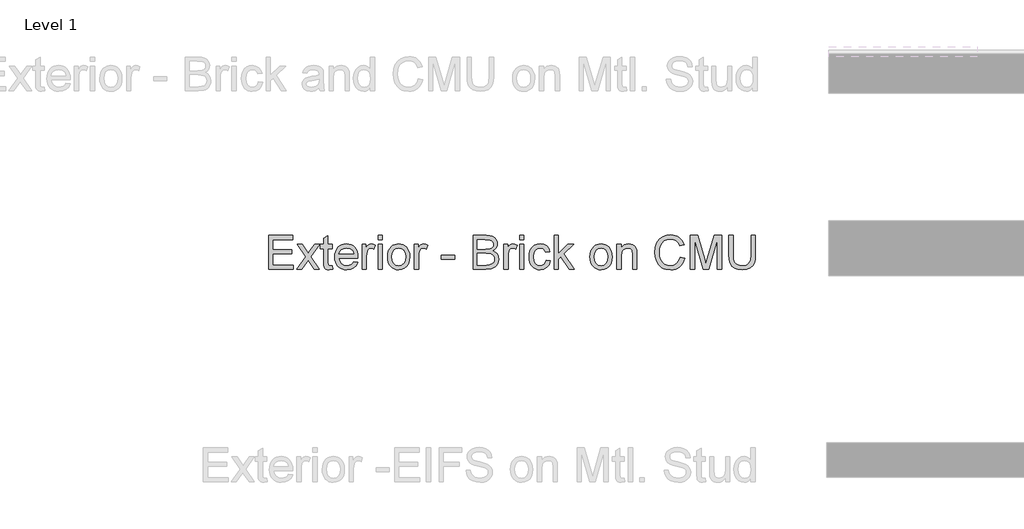
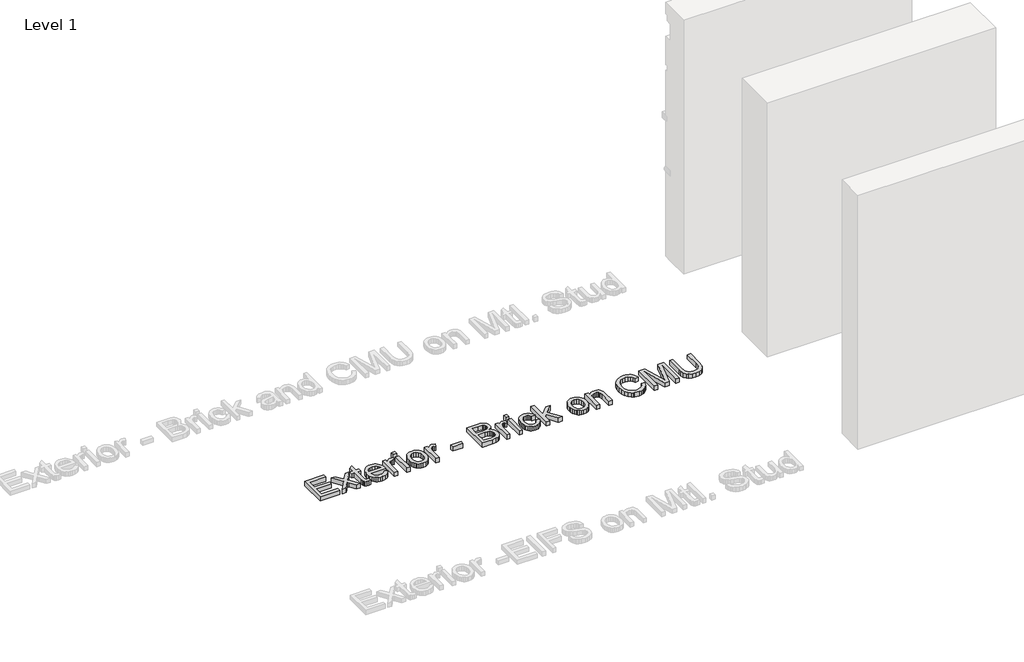
# One storey, part 25 of 42: 1 proxy.
"""IFC4 building model written with IfcOpenShell, lengths in millimetres."""

import ifcopenshell
import ifcopenshell.guid

model = None  # the IFC model being written
_history = None  # IfcOwnerHistory: only IFC2X3 demands one
_inside = {}  # id of a spatial element -> (the spatial element, [elements in it])
_under = {}  # id of a project, library or spatial element -> (it, [spatial elements below it])
_declared = {}  # id of a project -> (the project, [libraries it declares])
_typed = {}  # id of a type object -> (the type object, [elements of that type])
_made_of = {}  # id of a material, layer set ... -> (it, [elements and type objects made of it])


def new_model(schema):
    """Start an empty IFC model of exactly this schema.

    Asked for "IFC4X3", IfcOpenShell would pick the latest addendum, in which some entities
    have other attributes; the version numbers below select the first issue.
    IFC2X3 requires an IfcOwnerHistory on every rooted entity: one is made here for all.
    """
    global model, _history
    if schema == "IFC4X3":
        model = ifcopenshell.file(schema_version=(4, 3, 0, 0))
    else:
        model = ifcopenshell.file(schema=schema)
    _inside.clear()
    _under.clear()
    _declared.clear()
    _typed.clear()
    _made_of.clear()
    _history = None
    if model.schema == "IFC2X3":
        org = make("IfcOrganization", Name="unknown")
        user = make(
            "IfcPersonAndOrganization",
            ThePerson=make("IfcPerson", FamilyName="unknown"),
            TheOrganization=org,
        )
        app = make(
            "IfcApplication",
            ApplicationDeveloper=org,
            Version="unknown",
            ApplicationFullName="unknown",
            ApplicationIdentifier="unknown",
        )
        _history = make(
            "IfcOwnerHistory",
            OwningUser=user,
            OwningApplication=app,
            ChangeAction="ADDED",
            CreationDate=0,
        )
    return model


def make(cls, **values):
    """One entity of the class cls with the attributes given. An attribute that is None is left unset."""
    return model.create_entity(
        cls, **{name: value for name, value in values.items() if value is not None}
    )


def rooted(cls, **values):
    """An entity with a GlobalId (a new one), such as an element, a storey or a relation."""
    return make(cls, GlobalId=ifcopenshell.guid.new(), OwnerHistory=_history, **values)


def si_unit(unit_type, name, prefix=None):
    """IfcSIUnit, for example si_unit("LENGTHUNIT", "METRE", prefix="MILLI")."""
    return make("IfcSIUnit", UnitType=unit_type, Prefix=prefix, Name=name)


def assignment(units):
    """IfcUnitAssignment: the units of a project."""
    return None if units is None else make("IfcUnitAssignment", Units=units)


def point(xyz):
    """IfcCartesianPoint."""
    return None if xyz is None else make("IfcCartesianPoint", Coordinates=xyz)


def direction(xyz):
    """IfcDirection."""
    return None if xyz is None else make("IfcDirection", DirectionRatios=xyz)


def frame(location, z_axis=None, x_axis=None):
    """IfcAxis2Placement3D, a coordinate frame: its origin and axes. An axis left out is left unset."""
    return make(
        "IfcAxis2Placement3D",
        Location=point(location),
        Axis=direction(z_axis),
        RefDirection=direction(x_axis),
    )


def origin():
    """The frame at (0, 0, 0) with its axes left unset."""
    return frame((0.0, 0.0, 0.0))


def origin_with_axes():
    """The frame at (0, 0, 0) with the z axis (0, 0, 1) and the x axis (1, 0, 0) written out."""
    return frame((0.0, 0.0, 0.0), z_axis=(0.0, 0.0, 1.0), x_axis=(1.0, 0.0, 0.0))


def place(relative_to, where):
    """IfcLocalPlacement: puts the frame where relative to a parent placement (None: the world)."""
    return make(
        "IfcLocalPlacement", PlacementRelTo=relative_to, RelativePlacement=where
    )


def context(
    kind, dimensions, precision=None, world=None, true_north=None, identifier=None
):
    """IfcGeometricRepresentationContext, for example the 3D "Model" context."""
    return make(
        "IfcGeometricRepresentationContext",
        ContextIdentifier=identifier,
        ContextType=kind,
        CoordinateSpaceDimension=dimensions,
        Precision=precision,
        WorldCoordinateSystem=world,
        TrueNorth=true_north,
    )


def project(units=None, contexts=None):
    """IfcProject with its units and contexts."""
    return rooted(
        "IfcProject",
        Name="project",
        RepresentationContexts=contexts,
        UnitsInContext=assignment(units),
    )


def spatial(cls, under=None, at=None, **own):
    """A site, building, storey or space (cls), placed at a placement, below another one or the project."""
    s = rooted(cls, ObjectPlacement=at, **own)
    if under is not None:
        _under.setdefault(under.id(), (under, []))[1].append(s)
    return s


def polyline(points):
    """IfcPolyline through the points."""
    return make("IfcPolyline", Points=[point(p) for p in points])


def outline(outer, holes=None, kind="AREA"):
    """IfcArbitraryClosedProfileDef: a profile drawn as a closed curve; with holes, ...WithVoids."""
    if holes is None:
        return make("IfcArbitraryClosedProfileDef", ProfileType=kind, OuterCurve=outer)
    return make(
        "IfcArbitraryProfileDefWithVoids",
        ProfileType=kind,
        OuterCurve=outer,
        InnerCurves=holes,
    )


def extrude(swept, where, along, depth):
    """IfcExtrudedAreaSolid: the profile swept, set in the frame where, extruded along a direction by depth."""
    return make(
        "IfcExtrudedAreaSolid",
        SweptArea=swept,
        Position=where,
        ExtrudedDirection=direction(along),
        Depth=depth,
    )


def shape(context_of_items, identifier, shape_type, items):
    """IfcShapeRepresentation: the items that make up one representation, for example the "Body"."""
    return make(
        "IfcShapeRepresentation",
        ContextOfItems=context_of_items,
        RepresentationIdentifier=identifier,
        RepresentationType=shape_type,
        Items=items,
    )


def made_of(thing, what):
    """Note that an element or type object is made of a material, layer set ...; save() writes the relation."""
    if what is not None:
        _made_of.setdefault(what.id(), (what, []))[1].append(thing)
    return thing


def element(
    cls,
    number,
    at=None,
    inside=None,
    cuts=None,
    type_object=None,
    material=None,
    context=None,
    identifier="Body",
    shape_type=None,
    held_by="IfcProductDefinitionShape",
    body=None,
    shapes=None,
    **own,
):
    """One element of the class cls, such as IfcWall. Its Tag is "e" and its number.

    at: its placement. inside: the storey or other place that contains it. cuts: it is an
    opening in that element (IfcRelVoidsElement). A single representation is given by context,
    identifier, shape_type and body (its items); several are given by shapes. held_by: the class
    of the entity that holds the representations. save() writes the other relations.
    """
    e = rooted(cls, Tag="e%d" % number, ObjectPlacement=at, **own)
    if body is not None:
        shapes = [shape(context, identifier, shape_type, body)]
    if shapes is not None:
        e.Representation = make(held_by, Representations=shapes)
    if inside is not None:
        _inside.setdefault(inside.id(), (inside, []))[1].append(e)
    if cuts is not None:
        rooted(
            "IfcRelVoidsElement", RelatingBuildingElement=cuts, RelatedOpeningElement=e
        )
    if type_object is not None:
        _typed.setdefault(type_object.id(), (type_object, []))[1].append(e)
    return made_of(e, material)


def aggregate(whole, parts):
    """IfcRelAggregates: a whole, such as a stair, and the parts it consists of."""
    return rooted("IfcRelAggregates", RelatingObject=whole, RelatedObjects=parts)


def save(model, path):
    """Write the relations noted so far, then the file.

    IfcRelAggregates (storeys below a building ...), IfcRelContainedInSpatialStructure (elements
    in a storey), IfcRelDefinesByType, IfcRelAssociatesMaterial and IfcRelDeclares: one each for
    every whole, place, type object, material and project.
    """
    for whole, parts in _under.values():
        aggregate(whole, parts)
    for where, things in _inside.values():
        rooted(
            "IfcRelContainedInSpatialStructure",
            RelatedElements=things,
            RelatingStructure=where,
        )
    for kind, things in _typed.values():
        rooted("IfcRelDefinesByType", RelatedObjects=things, RelatingType=kind)
    for what, things in _made_of.values():
        rooted("IfcRelAssociatesMaterial", RelatedObjects=things, RelatingMaterial=what)
    for by, libraries in _declared.values():
        rooted("IfcRelDeclares", RelatingContext=by, RelatedDefinitions=libraries)
    model.write(path)


model = new_model("IFC4")

# Units and contexts
model_context = context("Model", 3, world=origin())
ifc_project = project(units=[si_unit("LENGTHUNIT", "METRE", prefix="MILLI")], contexts=[model_context])

# Site, building, storey
site = spatial("IfcSite", under=ifc_project)
building = spatial("IfcBuilding", under=site)
storey = spatial("IfcBuildingStorey", under=building, Name="Level 1", Elevation=0.0)

# Proxy
placement = place(None, origin())
element("IfcBuildingElementProxy", 1, Name="8\" Arial", ObjectType="8\" Arial", at=placement, inside=storey, context=model_context, shape_type="SweptSolid", body=[
    extrude(outline(polyline([(-4360.2631127, 8341.2295096), (-4360.2631127, 8645.7966037), (-4141.3555139, 8645.7966037), (-4141.3555139, 8607.7257169), (-4322.192226, 8607.7257169), (-4322.192226, 8517.3073608), (-4150.8732355, 8517.3073608), (-4150.8732355, 8479.2364741), (-4322.192226, 8479.2364741), (-4322.192226, 8379.3003963), (-4136.596653, 8379.3003963), (-4136.596653, 8341.2295096), (-4360.2631127, 8341.2295096)])), origin_with_axes(), (0.0, 0.0, 1.0), 50.8),
    extrude(outline(polyline([(-4108.0434879, 8341.2295096), (-4026.6967104, 8453.657597), (-4103.2846271, 8564.8959693), (-4057.4805915, 8564.8959693), (-4020.5250627, 8511.3587848), (-4003.2741922, 8486.0773366), (-3988.3283948, 8506.7486383), (-3946.2422192, 8564.8959693), (-3900.4381836, 8564.8959693), (-3980.8926747, 8453.657597), (-3903.4124716, 8341.2295096), (-3949.2165072, 8341.2295096), (-3995.8384721, 8408.820205), (-4004.3895502, 8421.1635003), (-4062.2394523, 8341.2295096), (-4108.0434879, 8341.2295096)])), origin_with_axes(), (0.0, 0.0, 1.0), 50.8),
    extrude(outline(polyline([(-3789.1998113, 8372.9800343), (-3784.4409505, 8340.1141516), (-3812.9197584, 8336.4706487), (-3831.1930404, 8338.0507393), (-3844.8189975, 8342.7910108), (-3854.448255, 8350.0966058), (-3860.7314384, 8359.3726666), (-3864.1890482, 8375.3036968), (-3865.3415849, 8402.5742002), (-3865.3415849, 8526.8250825), (-3893.8947499, 8526.8250825), (-3893.8947499, 8564.8959693), (-3865.3415849, 8564.8959693), (-3865.3415849, 8619.251083), (-3827.2706981, 8641.6326004), (-3827.2706981, 8564.8959693), (-3789.1998113, 8564.8959693), (-3789.1998113, 8526.8250825), (-3827.2706981, 8526.8250825), (-3827.2706981, 8403.6895582), (-3825.2630537, 8384.0592572), (-3818.7567986, 8377.1068589), (-3805.7814671, 8374.5415355), (-3789.1998113, 8372.9800343)])), origin_with_axes(), (0.0, 0.0, 1.0), 50.8),
    extrude(outline(polyline([(-3594.5326599, 8407.8535614), (-3557.2053452, 8403.0947006), (-3570.6547038, 8374.9690894), (-3592.1160509, 8353.9445909), (-3621.1060645, 8340.8391343), (-3657.1414229, 8336.4706487), (-3680.7637761, 8338.355139), (-3701.8115112, 8344.00861), (-3720.2846283, 8353.4310615), (-3736.1831272, 8366.6224936), (-3748.9679184, 8383.2157677), (-3758.0999121, 8402.843745), (-3763.5791084, 8425.5064256), (-3765.4055071, 8451.2038094), (-3763.5605191, 8477.7725667), (-3758.0255549, 8501.1904376), (-3748.8006147, 8521.4574221), (-3735.8856984, 8538.5735202), (-3720.0290254, 8552.1715933), (-3701.9788149, 8561.8845027), (-3681.735067, 8567.7122483), (-3659.2977817, 8569.6548301), (-3637.5831554, 8567.7168956), (-3617.9458835, 8561.903092), (-3600.3859658, 8552.2134193), (-3584.9034024, 8538.6478774), (-3572.265002, 8521.5689579), (-3563.2375731, 8501.339152), (-3557.8211157, 8477.9584597), (-3556.0156299, 8451.426881), (-3556.2387015, 8441.1655873), (-3727.3346204, 8441.1655873), (-3720.7447134, 8412.6681902), (-3705.4364247, 8391.7180489), (-3683.3430415, 8378.8356638), (-3656.3978509, 8374.5415355), (-3636.1355137, 8376.5305906), (-3619.0705361, 8382.497756), (-3605.2029182, 8392.8148176), (-3594.5326599, 8407.8535614)]), holes=[polyline([(-3727.3346204, 8479.2364741), (-3594.0865167, 8479.2364741), (-3599.2357528, 8499.3500969), (-3609.3297428, 8513.7382152), (-3631.5253673, 8527.1225113), (-3659.4464961, 8531.5839434), (-3685.109025, 8528.0240924), (-3706.3287112, 8517.3445394), (-3721.0793208, 8500.6978211), (-3727.3346204, 8479.2364741)])]), origin_with_axes(), (0.0, 0.0, 1.0), 50.8),
    extrude(outline(polyline([(-3517.9447432, 8341.2295096), (-3517.9447432, 8564.8959693), (-3484.6327173, 8564.8959693), (-3484.6327173, 8531.807015), (-3472.3266006, 8550.9911728), (-3460.9871274, 8562.2934673), (-3449.6104757, 8567.8144894), (-3437.1928232, 8569.6548301), (-3418.231737, 8566.7177207), (-3398.9732221, 8557.9063924), (-3411.6883034, 8523.7764373), (-3425.0725995, 8529.6320669), (-3438.4568956, 8531.5839434), (-3449.8242527, 8529.7064241), (-3459.9833052, 8524.0738661), (-3468.1904813, 8515.1138234), (-3473.7022088, 8503.2538499), (-3478.3309445, 8481.9876905), (-3479.8738564, 8458.7882439), (-3479.8738564, 8341.2295096), (-3517.9447432, 8341.2295096)])), origin_with_axes(), (0.0, 0.0, 1.0), 50.8),
    extrude(outline(polyline([(-3375.1789178, 8607.7257169), (-3375.1789178, 8645.7966037), (-3337.1080311, 8645.7966037), (-3337.1080311, 8607.7257169), (-3375.1789178, 8607.7257169)])), origin_with_axes(), (0.0, 0.0, 1.0), 50.8),
    extrude(outline(polyline([(-3375.1789178, 8341.2295096), (-3375.1789178, 8564.8959693), (-3337.1080311, 8564.8959693), (-3337.1080311, 8341.2295096), (-3375.1789178, 8341.2295096)])), origin_with_axes(), (0.0, 0.0, 1.0), 50.8),
    extrude(outline(polyline([(-3289.5194226, 8453.0627394), (-3287.4606576, 8482.0295164), (-3281.2843627, 8506.9902992), (-3270.9905377, 8527.9450879), (-3256.5791827, 8544.8938823), (-3242.0702339, 8555.726797), (-3226.0555518, 8563.4645932), (-3208.5351364, 8568.1072709), (-3189.5089877, 8569.6548301), (-3168.5054022, 8567.7703398), (-3149.5141084, 8562.1168689), (-3132.5351063, 8552.6944174), (-3117.568396, 8539.5029853), (-3105.3529021, 8522.9887157), (-3096.6275494, 8503.597752), (-3091.3923377, 8481.330094), (-3089.6472671, 8456.1857419), (-3092.733091, 8417.7244798), (-3101.9905625, 8388.446332), (-3117.1501368, 8366.5202525), (-3137.942269, 8350.1151951), (-3162.6381543, 8339.8817853), (-3189.5089877, 8336.4706487), (-3210.8192967, 8338.3481681), (-3229.9871888, 8343.980726), (-3247.0126641, 8353.3683226), (-3261.8957226, 8366.5109578), (-3273.9810913, 8383.1855601), (-3282.6134976, 8403.1690578), (-3287.7929414, 8426.4614509), (-3289.5194226, 8453.0627394)]), holes=[polyline([(-3251.4485359, 8453.1370966), (-3247.0428717, 8418.6818288), (-3233.8258793, 8394.1346579), (-3213.9353281, 8379.4398161), (-3189.5089877, 8374.5415355), (-3165.1941831, 8379.4677), (-3145.3408105, 8394.2461937), (-3132.123818, 8419.1186773), (-3127.7181539, 8454.3268119), (-3132.151702, 8487.7782575), (-3145.4523463, 8511.990821), (-3165.3336028, 8526.6856628), (-3189.5089877, 8531.5839434), (-3213.9353281, 8526.7042521), (-3233.8258793, 8512.0651782), (-3247.0428717, 8487.5737752), (-3251.4485359, 8453.1370966)])]), origin_with_axes(), (0.0, 0.0, 1.0), 50.8),
    extrude(outline(polyline([(-3046.8175195, 8341.2295096), (-3046.8175195, 8564.8959693), (-3013.5054936, 8564.8959693), (-3013.5054936, 8531.807015), (-3001.1993769, 8550.9911728), (-2989.8599038, 8562.2934673), (-2978.4832521, 8567.8144894), (-2966.0655996, 8569.6548301), (-2947.1045134, 8566.7177207), (-2927.8459984, 8557.9063924), (-2940.5610797, 8523.7764373), (-2953.9453759, 8529.6320669), (-2967.329672, 8531.5839434), (-2978.6970291, 8529.7064241), (-2988.8560816, 8524.0738661), (-2997.0632576, 8515.1138234), (-3002.5749851, 8503.2538499), (-3007.2037209, 8481.9876905), (-3008.7466328, 8458.7882439), (-3008.7466328, 8341.2295096), (-3046.8175195, 8341.2295096)])), origin_with_axes(), (0.0, 0.0, 1.0), 50.8),
    extrude(outline(polyline([(-2804.1156165, 8431.6478656), (-2804.1156165, 8469.7187524), (-2685.1440953, 8469.7187524), (-2685.1440953, 8431.6478656), (-2804.1156165, 8431.6478656)])), origin_with_axes(), (0.0, 0.0, 1.0), 50.8),
    extrude(outline(polyline([(-2518.5839658, 8341.2295096), (-2518.5839658, 8645.7966037), (-2402.3636611, 8645.7966037), (-2370.3993594, 8643.556593), (-2345.4432239, 8636.836561), (-2326.3148341, 8625.4692039), (-2311.8337692, 8609.2872181), (-2302.7157175, 8590.2517747), (-2299.6763669, 8570.3240449), (-2302.2323957, 8551.9857003), (-2309.900482, 8534.7441244), (-2322.7363938, 8519.6589073), (-2340.7958989, 8507.7896392), (-2319.223016, 8496.5245233), (-2303.2826911, 8479.3851885), (-2293.4396567, 8457.5055822), (-2290.1586452, 8432.0196516), (-2292.3986559, 8410.7813762), (-2299.1186879, 8391.0860127), (-2309.1476153, 8374.3370532), (-2321.3143123, 8361.93799), (-2336.2136364, 8352.959358), (-2354.4404452, 8346.4716922), (-2403.2559475, 8341.2295096), (-2518.5839658, 8341.2295096)]), holes=[polyline([(-2480.513079, 8522.0662217), (-2410.9890964, 8522.0662217), (-2370.3900648, 8525.3379385), (-2356.1785448, 8530.9797911), (-2345.9637243, 8539.4286281), (-2339.8013713, 8550.5543242), (-2337.7472537, 8564.2267545), (-2339.6619516, 8577.4995148), (-2345.4060453, 8589.0620595), (-2354.7192847, 8598.0871648), (-2367.3414195, 8603.7476067), (-2416.2684576, 8607.7257169), (-2480.513079, 8607.7257169), (-2480.513079, 8522.0662217)]), polyline([(-2480.513079, 8379.3003963), (-2402.4380183, 8379.3003963), (-2374.182282, 8380.7875404), (-2350.276442, 8389.0783682), (-2334.4383582, 8405.9946314), (-2329.7817385, 8417.9475514), (-2328.229532, 8431.6478656), (-2330.0512834, 8447.5603066), (-2335.5165376, 8461.2420315), (-2345.0621433, 8471.9401738), (-2359.1249489, 8478.9018667), (-2379.043384, 8482.7219679), (-2406.1558783, 8483.9953349), (-2480.513079, 8483.9953349), (-2480.513079, 8379.3003963)])]), origin_with_axes(), (0.0, 0.0, 1.0), 50.8),
    extrude(outline(polyline([(-2242.5700368, 8341.2295096), (-2242.5700368, 8564.8959693), (-2209.2580109, 8564.8959693), (-2209.2580109, 8531.807015), (-2196.9518941, 8550.9911728), (-2185.612421, 8562.2934673), (-2174.2357693, 8567.8144894), (-2161.8181168, 8569.6548301), (-2142.8570306, 8566.7177207), (-2123.5985157, 8557.9063924), (-2136.313597, 8523.7764373), (-2149.6978931, 8529.6320669), (-2163.0821892, 8531.5839434), (-2174.4495463, 8529.7064241), (-2184.6085988, 8524.0738661), (-2192.8157749, 8515.1138234), (-2198.3275024, 8503.2538499), (-2202.9562381, 8481.9876905), (-2204.49915, 8458.7882439), (-2204.49915, 8341.2295096), (-2242.5700368, 8341.2295096)])), origin_with_axes(), (0.0, 0.0, 1.0), 50.8),
    extrude(outline(polyline([(-2099.8042114, 8341.2295096), (-2099.8042114, 8564.8959693), (-2061.7333247, 8564.8959693), (-2061.7333247, 8341.2295096), (-2099.8042114, 8341.2295096)])), origin_with_axes(), (0.0, 0.0, 1.0), 50.8),
    extrude(outline(polyline([(-2099.8042114, 8607.7257169), (-2099.8042114, 8645.7966037), (-2061.7333247, 8645.7966037), (-2061.7333247, 8607.7257169), (-2099.8042114, 8607.7257169)])), origin_with_axes(), (0.0, 0.0, 1.0), 50.8),
    extrude(outline(polyline([(-1861.8611692, 8422.130144), (-1823.7902824, 8417.3712831), (-1834.4047728, 8383.5108728), (-1854.3510919, 8357.9227011), (-1881.7517204, 8341.8336618), (-1914.7291389, 8336.4706487), (-1936.0812738, 8338.3411971), (-1955.2259293, 8343.9528421), (-1972.1631054, 8353.3055837), (-1986.8928022, 8366.399422), (-1998.8155146, 8382.9880488), (-2007.3317377, 8402.8251557), (-2012.4414716, 8425.9107429), (-2014.1447162, 8452.2448102), (-2011.2354907, 8486.1238098), (-2002.5078143, 8515.4856094), (-1987.8222672, 8539.1962618), (-1967.0394296, 8556.1218196), (-1942.1762406, 8566.2715775), (-1915.2496393, 8569.6548301), (-1883.0808553, 8565.0075051), (-1857.3625585, 8551.06553), (-1838.9126781, 8528.5724768), (-1828.5491433, 8498.2719175), (-1866.62003, 8493.5130566), (-1873.525955, 8510.1225963), (-1884.2798652, 8522.0290431), (-1898.2869029, 8529.1952183), (-1914.9522105, 8531.5839434), (-1939.5551493, 8526.8808504), (-1959.0832091, 8512.7715716), (-1971.8261744, 8488.4939456), (-1976.0738295, 8453.285811), (-1971.9191209, 8417.6036494), (-1959.4549951, 8393.2423715), (-1940.280132, 8379.2167445), (-1915.9932113, 8374.5415355), (-1896.2792585, 8377.4600556), (-1880.115862, 8386.215616), (-1868.3581296, 8401.0312883), (-1861.8611692, 8422.130144)])), origin_with_axes(), (0.0, 0.0, 1.0), 50.8),
    extrude(outline(polyline([(-1790.4782565, 8341.2295096), (-1790.4782565, 8645.7966037), (-1752.4073698, 8645.7966037), (-1752.4073698, 8482.1364049), (-1667.0453034, 8564.8959693), (-1614.4004053, 8564.8959693), (-1700.8034725, 8481.0954041), (-1609.6415444, 8341.2295096), (-1654.1071504, 8341.2295096), (-1728.0925651, 8454.6242407), (-1752.4073698, 8431.053008), (-1752.4073698, 8341.2295096), (-1790.4782565, 8341.2295096)])), origin_with_axes(), (0.0, 0.0, 1.0), 50.8),
    extrude(outline(polyline([(-1466.8757191, 8453.0627394), (-1464.8169541, 8482.0295164), (-1458.6406591, 8506.9902992), (-1448.3468341, 8527.9450879), (-1433.9354792, 8544.8938823), (-1419.4265304, 8555.726797), (-1403.4118483, 8563.4645932), (-1385.8914329, 8568.1072709), (-1366.8652841, 8569.6548301), (-1345.8616986, 8567.7703398), (-1326.8704048, 8562.1168689), (-1309.8914028, 8552.6944174), (-1294.9246924, 8539.5029853), (-1282.7091986, 8522.9887157), (-1273.9838458, 8503.597752), (-1268.7486341, 8481.330094), (-1267.0035636, 8456.1857419), (-1270.0893874, 8417.7244798), (-1279.3468589, 8388.446332), (-1294.5064332, 8366.5202525), (-1315.2985654, 8350.1151951), (-1339.9944507, 8339.8817853), (-1366.8652841, 8336.4706487), (-1388.1755931, 8338.3481681), (-1407.3434853, 8343.980726), (-1424.3689606, 8353.3683226), (-1439.252019, 8366.5109578), (-1451.3373878, 8383.1855601), (-1459.9697941, 8403.1690578), (-1465.1492378, 8426.4614509), (-1466.8757191, 8453.0627394)]), holes=[polyline([(-1428.8048323, 8453.1370966), (-1424.3991682, 8418.6818288), (-1411.1821757, 8394.1346579), (-1391.2916246, 8379.4398161), (-1366.8652841, 8374.5415355), (-1342.5504795, 8379.4677), (-1322.6971069, 8394.2461937), (-1309.4801145, 8419.1186773), (-1305.0744503, 8454.3268119), (-1309.5079984, 8487.7782575), (-1322.8086427, 8511.990821), (-1342.6898992, 8526.6856628), (-1366.8652841, 8531.5839434), (-1391.2916246, 8526.7042521), (-1411.1821757, 8512.0651782), (-1424.3991682, 8487.5737752), (-1428.8048323, 8453.1370966)])]), origin_with_axes(), (0.0, 0.0, 1.0), 50.8),
    extrude(outline(polyline([(-1224.173816, 8341.2295096), (-1224.173816, 8564.8959693), (-1186.1029292, 8564.8959693), (-1186.1029292, 8533.665945), (-1172.8766421, 8549.4110822), (-1156.9920851, 8560.6576089), (-1138.4492582, 8567.4055248), (-1117.2481614, 8569.6548301), (-1098.4822628, 8567.8423734), (-1081.2964548, 8562.4050031), (-1066.9641044, 8554.0212287), (-1056.7585786, 8543.3695597), (-1045.3447483, 8515.3740736), (-1043.3371039, 8478.5672593), (-1043.3371039, 8341.2295096), (-1081.4079906, 8341.2295096), (-1081.4079906, 8473.4366124), (-1085.7950655, 8507.1204244), (-1091.864472, 8517.1493518), (-1101.2985418, 8524.9289739), (-1113.3908816, 8529.920201), (-1127.4350979, 8531.5839434), (-1149.7329634, 8527.847494), (-1168.7405229, 8516.638146), (-1176.3365756, 8507.487563), (-1181.7623276, 8494.9816113), (-1186.1029292, 8459.9036019), (-1186.1029292, 8341.2295096), (-1224.173816, 8341.2295096)])), origin_with_axes(), (0.0, 0.0, 1.0), 50.8),
    extrude(outline(polyline([(-653.1105146, 8449.4935938), (-615.0396278, 8439.6784433), (-622.5729417, 8416.0026459), (-632.6065165, 8395.3150784), (-645.1403522, 8377.615741), (-660.1744487, 8362.9046336), (-677.3695513, 8351.3397652), (-696.3864054, 8343.079145), (-717.2250109, 8338.1227728), (-739.8853678, 8336.4706487), (-784.0442504, 8341.4711705), (-802.7148787, 8347.7218227), (-819.1129652, 8356.4727357), (-845.9930932, 8380.9548441), (-865.5862156, 8414.3969951), (-877.5484303, 8453.7133649), (-881.5358352, 8495.8181298), (-877.0279299, 8540.227968), (-863.504214, 8578.5776942), (-841.6710809, 8609.6497095), (-812.2349241, 8632.2264145), (-777.3242184, 8645.973202), (-739.0674386, 8650.5554645), (-717.2923971, 8649.0729678), (-697.3251651, 8644.6254777), (-679.1657425, 8637.2129943), (-662.8141293, 8626.8355175), (-648.5398704, 8613.7672395), (-636.6125107, 8598.2823524), (-619.7984887, 8560.0627512), (-657.8693754, 8550.9911728), (-671.0677786, 8578.7542926), (-689.0993997, 8597.7990306), (-712.1873106, 8608.813191), (-740.5545826, 8612.4845777), (-773.2531616, 8608.413521), (-800.1147004, 8596.2003508), (-820.497868, 8577.1277288), (-833.7613337, 8552.4783168), (-841.0390447, 8524.6129558), (-843.4649484, 8495.892487), (-840.5929015, 8460.7215311), (-831.9767609, 8430.309436), (-817.2912137, 8405.818033), (-796.2109474, 8388.4091534), (-770.9387938, 8378.00844), (-743.6775851, 8374.5415355), (-711.8991764, 8379.2632177), (-685.4187183, 8393.4282645), (-665.425926, 8416.8879613), (-653.1105146, 8449.4935938)])), origin_with_axes(), (0.0, 0.0, 1.0), 50.8),
    extrude(outline(polyline([(-562.6921586, 8341.2295096), (-562.6921586, 8645.7966037), (-497.1834647, 8645.7966037), (-434.8721305, 8431.1273652), (-422.3057636, 8386.2899732), (-408.6983959, 8434.8452253), (-347.4280625, 8645.7966037), (-281.9193687, 8645.7966037), (-281.9193687, 8341.2295096), (-319.9902555, 8341.2295096), (-319.9902555, 8607.7257169), (-396.503815, 8341.2295096), (-448.1077123, 8341.2295096), (-524.6212718, 8607.7257169), (-524.6212718, 8341.2295096), (-562.6921586, 8341.2295096)])), origin_with_axes(), (0.0, 0.0, 1.0), 50.8),
    extrude(outline(polyline([(-15.4231614, 8645.7966037), (22.6477254, 8645.7966037), (22.6477254, 8470.0905384), (20.0638126, 8428.9431225), (12.3120745, 8397.2576603), (-2.1689904, 8372.8127306), (-24.9408831, 8353.3869119), (-56.0593716, 8340.6997145), (-95.5802238, 8336.4706487), (-134.2366735, 8340.1513302), (-165.141385, 8351.1933745), (-188.303653, 8369.215701), (-203.7327722, 8393.8372291), (-212.4046807, 8426.8611208), (-215.2953169, 8470.0905384), (-215.2953169, 8645.7966037), (-177.2244301, 8645.7966037), (-177.2244301, 8471.428968), (-175.3469108, 8437.215361), (-169.7143529, 8413.3931729), (-159.5088271, 8396.895169), (-143.9124042, 8384.6541148), (-123.5757098, 8377.0696803), (-99.1493694, 8374.5415355), (-60.4278571, 8379.5420572), (-45.9328503, 8385.7927094), (-34.6816764, 8394.5436225), (-26.2560761, 8406.8497392), (-20.2377901, 8423.7660024), (-15.4231614, 8471.428968), (-15.4231614, 8645.7966037)])), origin_with_axes(), (0.0, 0.0, 1.0), 50.8),
])

save(model, "model.ifc")

# Revit data of these elements
# Element 1 (IfcBuildingElementProxy, "8\" Arial")
#   Phase Created = New Construction
